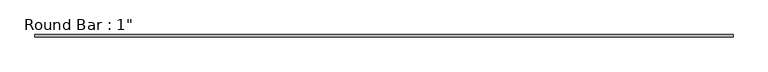
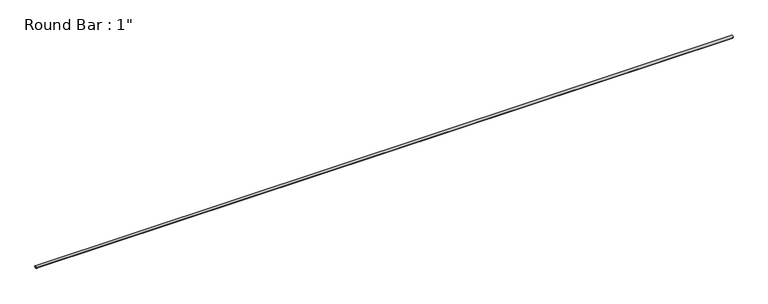
"""IFC4 building model written with IfcOpenShell, lengths in millimetres: member geometry."""

from ifc_helpers import new_model, si_unit, point, frame, origin, origin_2d, place, context, project, spatial, circle_curve, trimmed, segment, composite_curve, outline, extrude, source, transform, mapped, element, save


def member_52f726d1(model_context):
    return source(origin(), model_context, "Body", "SweptSolid", [
        extrude(outline(composite_curve([segment(trimmed(circle_curve(origin_2d(), 12.7), [point((-12.7, 0.0))], [point((12.7, 0.0))], False, "CARTESIAN"), True, "CONTINUOUS"), segment(trimmed(circle_curve(origin_2d(), 12.7), [point((12.7, 0.0))], [point((-12.7, 0.0))], False, "CARTESIAN"), True, "CONTINUOUS")], self_intersect=False)), frame((-3554.2056387, 0.0, 0.0), z_axis=(1.0, 0.0, 0.0), x_axis=(0.0, 1.0, 0.0)), (0.0, 0.0, 1.0), 7108.4112774),
    ])


if __name__ == "__main__":
    model = new_model("IFC4")
    model_context = context("Model", 3, world=origin())
    ifc_project = project(units=[si_unit("LENGTHUNIT", "METRE", prefix="MILLI")], contexts=[model_context])
    site = spatial("IfcSite", under=ifc_project)
    building = spatial("IfcBuilding", under=site)
    placement = place(None, origin())
    member_shape = member_52f726d1(model_context)
    element("IfcMember", 1, ObjectType="Round Bar : 1\"", at=placement, inside=building, context=model_context, shape_type="MappedRepresentation", body=[
        mapped(member_shape, transform((0.0, 0.0, 0.0), x_axis=(1.0, 0.0, 0.0), y_axis=(0.0, 1.0, 0.0), z_axis=(0.0, 0.0, 1.0))),
    ])
    save(model, "model.ifc")

# Revit data of these elements
# Type "Round Bar : 1\""
#   Assembly Code = "B10"
#   W = 0
#   Start Extension Calculation [instance default] = 10' - 0"
#   Start Extension [instance default] = -0' - 0 1/2"
#   End Extension Calculation [instance default] = 10' - 0"
#   End Extension [instance default] = -0' - 0 1/2"
#   Length [instance default] = 5' - 0"
#   d = 0' - 1"
#   A = 0 SF
#   Structural Material [instance default] = Metal - Steel - ASTM A36
# Element 1 (IfcMember, "Round Bar : 1\"")
#   Materials on its faces: "Metal - Steel - ASTM A36"
# Materials
#   "Metal - Steel - ASTM A36": class "Metal", colour RGB 199 199 199, transparency 0
